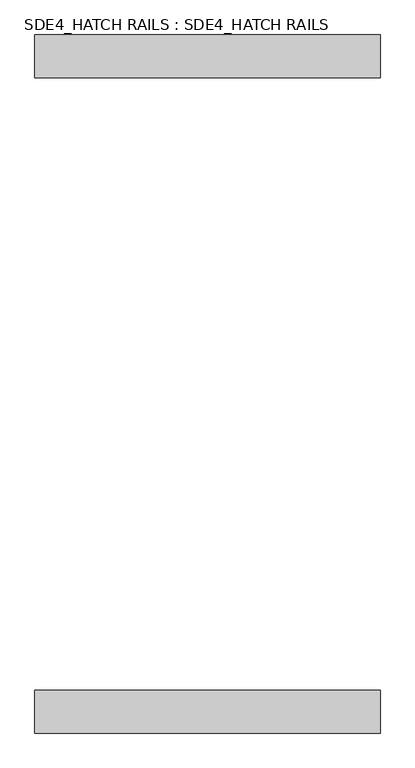
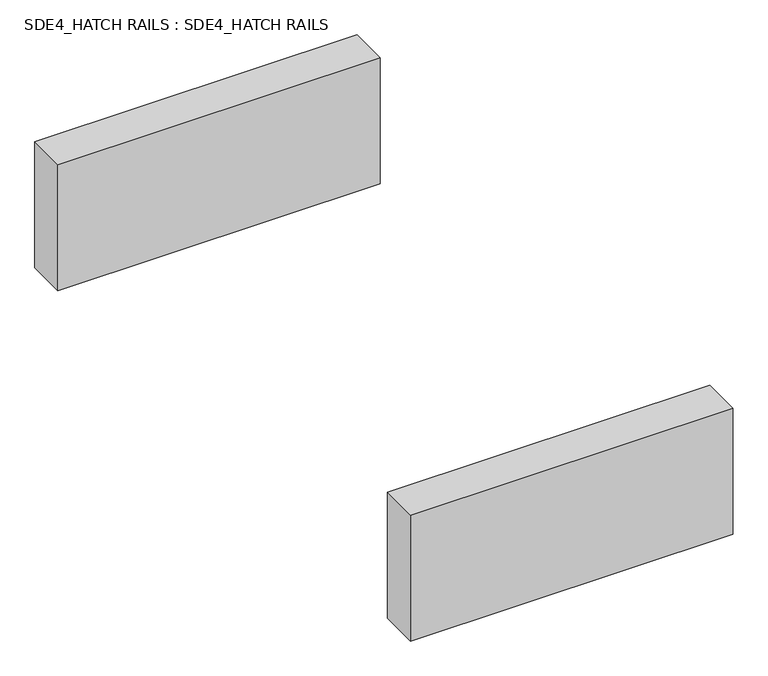
"""IFC4 building model written with IfcOpenShell, lengths in millimetres: proxy geometry, SDE4_HATCH RAILS : SDE4_HATCH RAILS."""

from ifc_helpers import new_model, si_unit, frame, origin, place, context, project, spatial, polyline, outline, extrude, source, transform, mapped, element, save


def sde4_hatch_rails_sde4_hatch_rails_605ecd68(model_context):
    return source(origin(), model_context, "Body", "SweptSolid", [
        extrude(outline(polyline([(65924.7995218, 25098.5988173), (66529.7995218, 25098.5988173), (66529.7995218, 25023.5988173), (65924.7995218, 25023.5988173), (65924.7995218, 25098.5988173)])), frame((0.0, 0.0, 148320.0), z_axis=(0.0, 0.0, 1.0), x_axis=(1.0, 0.0, 0.0)), (0.0, 0.0, 1.0), 250.0),
        extrude(outline(polyline([(65924.7995218, 23951.3985173), (66529.7995218, 23951.3985173), (66529.7995218, 23876.3985173), (65924.7995218, 23876.3985173), (65924.7995218, 23951.3985173)])), frame((0.0, 0.0, 148320.0), z_axis=(0.0, 0.0, 1.0), x_axis=(1.0, 0.0, 0.0)), (0.0, 0.0, 1.0), 250.0),
    ])


if __name__ == "__main__":
    model = new_model("IFC4")
    model_context = context("Model", 3, world=origin())
    ifc_project = project(units=[si_unit("LENGTHUNIT", "METRE", prefix="MILLI")], contexts=[model_context])
    site = spatial("IfcSite", under=ifc_project)
    building = spatial("IfcBuilding", under=site)
    placement = place(None, origin())
    sde4_hatch_rails_sde4_hatch_rails_shape = sde4_hatch_rails_sde4_hatch_rails_605ecd68(model_context)
    element("IfcBuildingElementProxy", 1, Name="SDE4_HATCH RAILS : SDE4_HATCH RAILS", ObjectType="SDE4_HATCH RAILS : SDE4_HATCH RAILS", at=placement, inside=building, context=model_context, shape_type="MappedRepresentation", body=[
        mapped(sde4_hatch_rails_sde4_hatch_rails_shape, transform((0.0, 0.0, 0.0), x_axis=(1.0, 0.0, 0.0), y_axis=(0.0, 1.0, 0.0), z_axis=(0.0, 0.0, 1.0))),
    ])
    save(model, "model.ifc")
